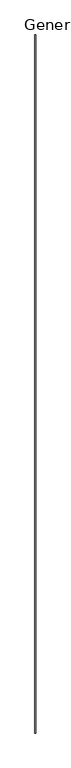
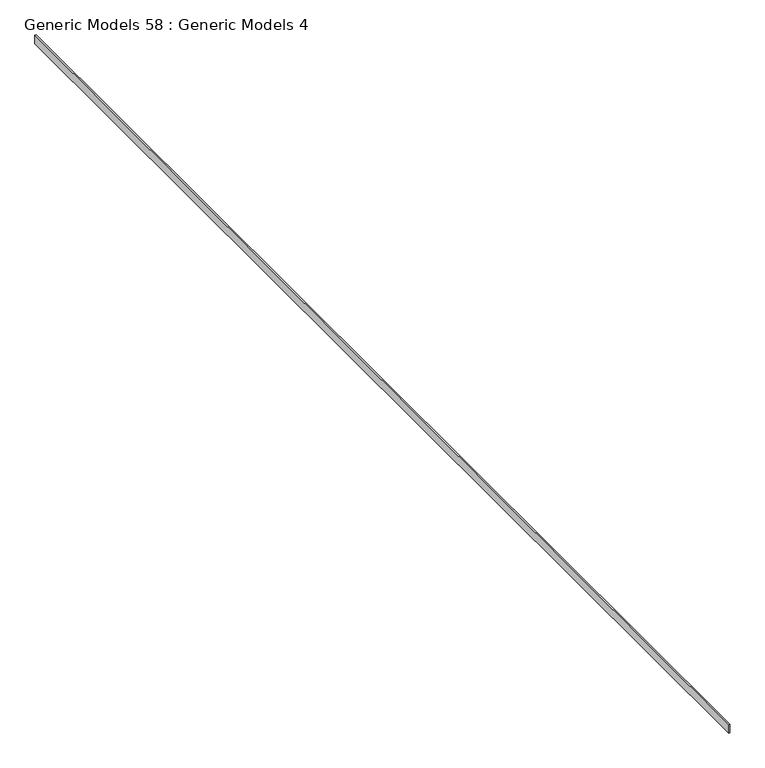
"""IFC4 building model written with IfcOpenShell, lengths in millimetres: proxy geometry, Generic Models 58 : Generic Models 4."""

from ifc_helpers import new_model, si_unit, frame, origin, place, context, project, spatial, polyline, outline, extrude, source, transform, mapped, element, save


def generic_models_58_generic_models_4_50999481(model_context):
    return source(origin(), model_context, "Body", "SweptSolid", [
        extrude(outline(polyline([(8346.0514146, -6864.9230338), (8327.0014146, -6864.9230338), (8327.0014146, 11778.6769662), (8346.0514146, 11778.6769662), (8346.0514146, -6864.9230338)])), frame((0.0, 0.0, 126778.6280968), z_axis=(0.0, 0.0, 1.0), x_axis=(1.0, 0.0, 0.0)), (0.0, 0.0, 1.0), 139.0309129),
    ])


if __name__ == "__main__":
    model = new_model("IFC4")
    model_context = context("Model", 3, world=origin())
    ifc_project = project(units=[si_unit("LENGTHUNIT", "METRE", prefix="MILLI")], contexts=[model_context])
    site = spatial("IfcSite", under=ifc_project)
    building = spatial("IfcBuilding", under=site)
    placement = place(None, origin())
    generic_models_58_generic_models_4_shape = generic_models_58_generic_models_4_50999481(model_context)
    element("IfcBuildingElementProxy", 1, Name="Generic Models 58 : Generic Models 4", ObjectType="Generic Models 58 : Generic Models 4", at=placement, inside=building, context=model_context, shape_type="MappedRepresentation", body=[
        mapped(generic_models_58_generic_models_4_shape, transform((0.0, 0.0, 0.0), x_axis=(1.0, 0.0, 0.0), y_axis=(0.0, 1.0, 0.0), z_axis=(0.0, 0.0, 1.0))),
    ])
    save(model, "model.ifc")

# Revit data of these elements
# Element 1 (IfcBuildingElementProxy, "Generic Models 58 : Generic Models 4")
#   Materials on its faces: "_CDX PLYWOOD - SEE STRUCT DWGs"
# Materials
#   "_CDX PLYWOOD - SEE STRUCT DWGs": class "Generic", colour RGB 98 75 74, transparency 0, Cost = 0
